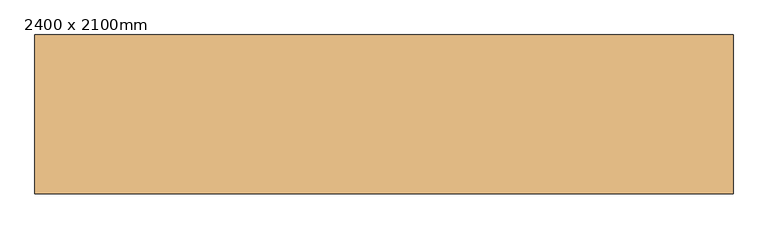
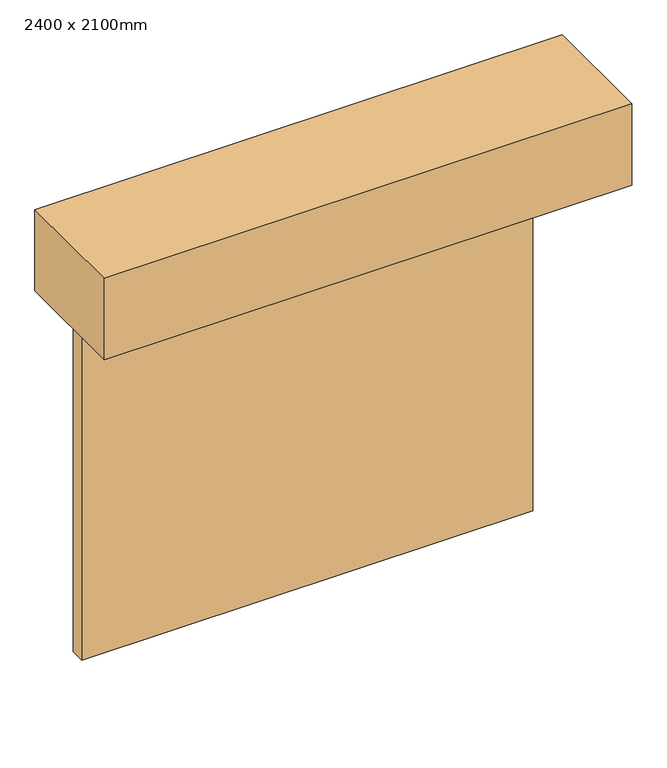
"""IFC4 building model written with IfcOpenShell, lengths in millimetres: door geometry, 滑升门 : 2400 x 2100mm."""

from ifc_helpers import new_model, si_unit, frame, origin, origin_with_axes, place, context, project, spatial, polyline, outline, extrude, source, transform, mapped, element, save


def door_2400_x_2100mm_76126092(model_context):
    return source(origin(), model_context, "Body", "SweptSolid", [
        extrude(outline(polyline([(1200.0, -120.0), (1200.0, -200.0), (-1200.0, -200.0), (-1200.0, -120.0), (1200.0, -120.0)])), origin_with_axes(), (0.0, 0.0, 1.0), 2100.0),
        extrude(outline(polyline([(1403.2, -758.8), (-1403.2, -758.8), (-1403.2, -120.0), (1403.2, -120.0), (1403.2, -758.8)])), frame((0.0, 0.0, 2100.0), z_axis=(0.0, 0.0, 1.0), x_axis=(1.0, 0.0, 0.0)), (0.0, 0.0, 1.0), 457.2),
    ])


if __name__ == "__main__":
    model = new_model("IFC4")
    model_context = context("Model", 3, world=origin())
    ifc_project = project(units=[si_unit("LENGTHUNIT", "METRE", prefix="MILLI")], contexts=[model_context])
    site = spatial("IfcSite", under=ifc_project)
    building = spatial("IfcBuilding", under=site)
    placement = place(None, origin())
    door_2400_x_2100mm_shape = door_2400_x_2100mm_76126092(model_context)
    element("IfcDoor", 1, ObjectType="滑升门 : 2400 x 2100mm", at=placement, inside=building, context=model_context, shape_type="MappedRepresentation", body=[
        mapped(door_2400_x_2100mm_shape, transform((0.0, 0.0, 0.0), x_axis=(1.0, 0.0, 0.0), y_axis=(0.0, 1.0, 0.0), z_axis=(0.0, 0.0, 1.0))),
    ])
    save(model, "model.ifc")

# Revit data of these elements
# Type "滑升门 : 2400 x 2100mm"
#   Type Mark = "M837"
#   Construction Type Id = "MDOOR"
#   Analytic Construction = "金属"
#   Thickness = 80 mm
#   Rough Width = 2400 mm
#   Rough Height = 2100 mm
#   Height = 2100 mm
#   Width = 2400 mm
#   Heat Transfer Coefficient (U) = 3.7021 W/(m²·K)
#   卷帘盒可见性 [instance default] = yes
#   Function = 1
#   卷帘箱材质 = none
#   门嵌板材质 = none
#   Visual Light Transmittance = 0
#   Solar Heat Gain Coefficient = 0
#   Wall Closure = (empty or 0)
